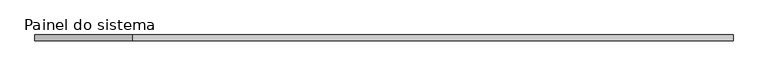
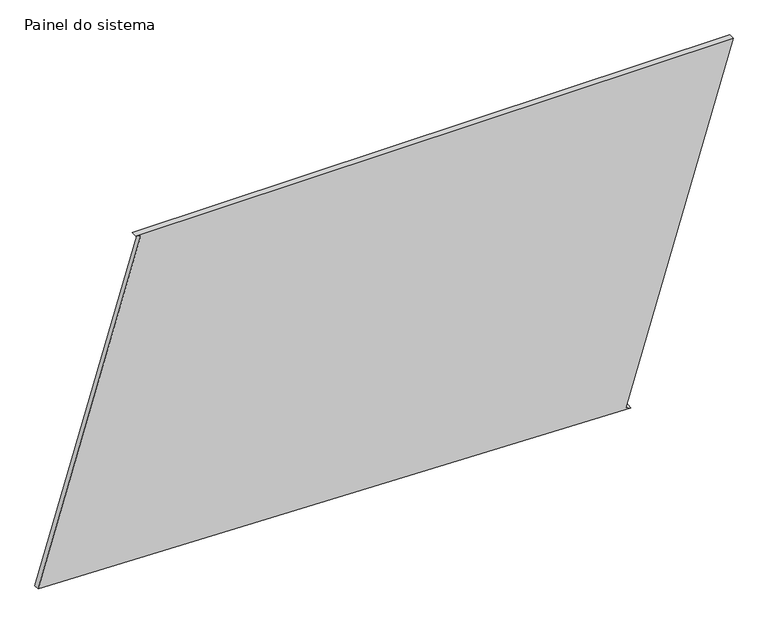
"""IFC4 building model written with IfcOpenShell, lengths in millimetres: plate geometry, Painel do sistema : Envidraçado."""

from ifc_helpers import new_model, si_unit, frame, origin, place, context, project, spatial, polyline, outline, extrude, source, transform, mapped, element, save


def painel_do_sistema_1f054f0c(model_context):
    return source(origin(), model_context, "Body", "SweptSolid", [
        extrude(outline(polyline([(0.0, 1093.0578611), (7.2712141, 1069.1386335), (1583.4223153, 1548.2733408), (1583.4223153, -1114.4683119), (1576.1511012, -1090.5490844), (70.4313529, -1548.2733408), (0.0, 1093.0578611)])), frame((0.0, 24.5, 0.0), z_axis=(0.0, 1.0, 0.0), x_axis=(0.0, 0.0, 1.0)), (0.0, 0.0, 1.0), 25.0),
    ])


if __name__ == "__main__":
    model = new_model("IFC4")
    model_context = context("Model", 3, world=origin())
    ifc_project = project(units=[si_unit("LENGTHUNIT", "METRE", prefix="MILLI")], contexts=[model_context])
    site = spatial("IfcSite", under=ifc_project)
    building = spatial("IfcBuilding", under=site)
    placement = place(None, origin())
    painel_do_sistema_shape = painel_do_sistema_1f054f0c(model_context)
    element("IfcPlate", 1, ObjectType="Painel do sistema : Envidraçado", at=placement, inside=building, context=model_context, shape_type="MappedRepresentation", body=[
        mapped(painel_do_sistema_shape, transform((0.0, 0.0, 0.0), x_axis=(1.0, 0.0, 0.0), y_axis=(0.0, 1.0, 0.0), z_axis=(0.0, 0.0, 1.0))),
    ])
    save(model, "model.ifc")

# Revit data of these elements
# Type "Painel do sistema : Envidraçado"
#   Construction Type Id = "GSP4R"
#   Analytic Construction = "Vidraça única Pilkington 1/8 pol"
#   Visual Light Transmittance = 0.9
#   Solar Heat Gain Coefficient = 0.86
#   Heat Transfer Coefficient (U) = 6.7069 W/(m²·K)
# Element 1 (IfcPlate, "Painel do sistema : Envidraçado")
#   Materials on its faces: "Vidro"
# Materials
#   "Vidro": class "Vidro", colour RGB 0 128 192, transparency 0.9, Description = "Vidro de sílica", Cost = 0
